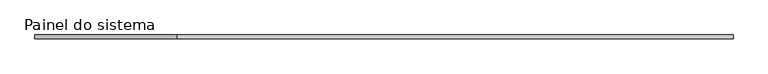
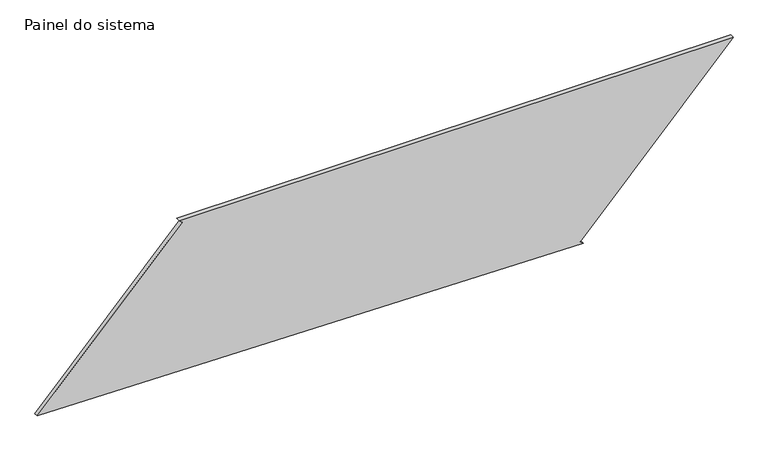
"""IFC4 building model written with IfcOpenShell, lengths in millimetres: plate geometry, Painel do sistema : Envidraçado."""

import ifcopenshell
import ifcopenshell.guid

model = None  # the IFC model being written
_history = None  # IfcOwnerHistory: only IFC2X3 demands one
_inside = {}  # id of a spatial element -> (the spatial element, [elements in it])
_under = {}  # id of a project, library or spatial element -> (it, [spatial elements below it])
_declared = {}  # id of a project -> (the project, [libraries it declares])
_typed = {}  # id of a type object -> (the type object, [elements of that type])
_made_of = {}  # id of a material, layer set ... -> (it, [elements and type objects made of it])


def new_model(schema):
    """Start an empty IFC model of exactly this schema.

    Asked for "IFC4X3", IfcOpenShell would pick the latest addendum, in which some entities
    have other attributes; the version numbers below select the first issue.
    IFC2X3 requires an IfcOwnerHistory on every rooted entity: one is made here for all.
    """
    global model, _history
    if schema == "IFC4X3":
        model = ifcopenshell.file(schema_version=(4, 3, 0, 0))
    else:
        model = ifcopenshell.file(schema=schema)
    _inside.clear()
    _under.clear()
    _declared.clear()
    _typed.clear()
    _made_of.clear()
    _history = None
    if model.schema == "IFC2X3":
        org = make("IfcOrganization", Name="unknown")
        user = make(
            "IfcPersonAndOrganization",
            ThePerson=make("IfcPerson", FamilyName="unknown"),
            TheOrganization=org,
        )
        app = make(
            "IfcApplication",
            ApplicationDeveloper=org,
            Version="unknown",
            ApplicationFullName="unknown",
            ApplicationIdentifier="unknown",
        )
        _history = make(
            "IfcOwnerHistory",
            OwningUser=user,
            OwningApplication=app,
            ChangeAction="ADDED",
            CreationDate=0,
        )
    return model


def make(cls, **values):
    """One entity of the class cls with the attributes given. An attribute that is None is left unset."""
    return model.create_entity(
        cls, **{name: value for name, value in values.items() if value is not None}
    )


def rooted(cls, **values):
    """An entity with a GlobalId (a new one), such as an element, a storey or a relation."""
    return make(cls, GlobalId=ifcopenshell.guid.new(), OwnerHistory=_history, **values)


def si_unit(unit_type, name, prefix=None):
    """IfcSIUnit, for example si_unit("LENGTHUNIT", "METRE", prefix="MILLI")."""
    return make("IfcSIUnit", UnitType=unit_type, Prefix=prefix, Name=name)


def assignment(units):
    """IfcUnitAssignment: the units of a project."""
    return None if units is None else make("IfcUnitAssignment", Units=units)


def point(xyz):
    """IfcCartesianPoint."""
    return None if xyz is None else make("IfcCartesianPoint", Coordinates=xyz)


def direction(xyz):
    """IfcDirection."""
    return None if xyz is None else make("IfcDirection", DirectionRatios=xyz)


def frame(location, z_axis=None, x_axis=None):
    """IfcAxis2Placement3D, a coordinate frame: its origin and axes. An axis left out is left unset."""
    return make(
        "IfcAxis2Placement3D",
        Location=point(location),
        Axis=direction(z_axis),
        RefDirection=direction(x_axis),
    )


def origin():
    """The frame at (0, 0, 0) with its axes left unset."""
    return frame((0.0, 0.0, 0.0))


def place(relative_to, where):
    """IfcLocalPlacement: puts the frame where relative to a parent placement (None: the world)."""
    return make(
        "IfcLocalPlacement", PlacementRelTo=relative_to, RelativePlacement=where
    )


def context(
    kind, dimensions, precision=None, world=None, true_north=None, identifier=None
):
    """IfcGeometricRepresentationContext, for example the 3D "Model" context."""
    return make(
        "IfcGeometricRepresentationContext",
        ContextIdentifier=identifier,
        ContextType=kind,
        CoordinateSpaceDimension=dimensions,
        Precision=precision,
        WorldCoordinateSystem=world,
        TrueNorth=true_north,
    )


def project(units=None, contexts=None):
    """IfcProject with its units and contexts."""
    return rooted(
        "IfcProject",
        Name="project",
        RepresentationContexts=contexts,
        UnitsInContext=assignment(units),
    )


def spatial(cls, under=None, at=None, **own):
    """A site, building, storey or space (cls), placed at a placement, below another one or the project."""
    s = rooted(cls, ObjectPlacement=at, **own)
    if under is not None:
        _under.setdefault(under.id(), (under, []))[1].append(s)
    return s


def polyline(points):
    """IfcPolyline through the points."""
    return make("IfcPolyline", Points=[point(p) for p in points])


def outline(outer, holes=None, kind="AREA"):
    """IfcArbitraryClosedProfileDef: a profile drawn as a closed curve; with holes, ...WithVoids."""
    if holes is None:
        return make("IfcArbitraryClosedProfileDef", ProfileType=kind, OuterCurve=outer)
    return make(
        "IfcArbitraryProfileDefWithVoids",
        ProfileType=kind,
        OuterCurve=outer,
        InnerCurves=holes,
    )


def extrude(swept, where, along, depth):
    """IfcExtrudedAreaSolid: the profile swept, set in the frame where, extruded along a direction by depth."""
    return make(
        "IfcExtrudedAreaSolid",
        SweptArea=swept,
        Position=where,
        ExtrudedDirection=direction(along),
        Depth=depth,
    )


def shape(context_of_items, identifier, shape_type, items):
    """IfcShapeRepresentation: the items that make up one representation, for example the "Body"."""
    return make(
        "IfcShapeRepresentation",
        ContextOfItems=context_of_items,
        RepresentationIdentifier=identifier,
        RepresentationType=shape_type,
        Items=items,
    )


def source(mapping_origin, context_of_items, identifier, shape_type, items):
    """IfcRepresentationMap: a shape defined once, which mapped items show again and again."""
    return make(
        "IfcRepresentationMap",
        MappingOrigin=mapping_origin,
        MappedRepresentation=shape(context_of_items, identifier, shape_type, items),
    )


def transform(
    local_origin,
    x_axis=None,
    y_axis=None,
    z_axis=None,
    scale=None,
    scale2=None,
    scale3=None,
    uniform=True,
):
    """IfcCartesianTransformationOperator3D, or its non-uniform kind. x_axis, y_axis, z_axis: its Axis1, 2, 3."""
    if uniform:
        return make(
            "IfcCartesianTransformationOperator3D",
            Axis1=direction(x_axis),
            Axis2=direction(y_axis),
            LocalOrigin=point(local_origin),
            Scale=scale,
            Axis3=direction(z_axis),
        )
    return make(
        "IfcCartesianTransformationOperator3DnonUniform",
        Axis1=direction(x_axis),
        Axis2=direction(y_axis),
        LocalOrigin=point(local_origin),
        Scale=scale,
        Axis3=direction(z_axis),
        Scale2=scale2,
        Scale3=scale3,
    )


def mapped(mapping_source, mapping_target):
    """IfcMappedItem: shows the shape of a source again, moved by a transform."""
    return make(
        "IfcMappedItem", MappingSource=mapping_source, MappingTarget=mapping_target
    )


def made_of(thing, what):
    """Note that an element or type object is made of a material, layer set ...; save() writes the relation."""
    if what is not None:
        _made_of.setdefault(what.id(), (what, []))[1].append(thing)
    return thing


def element(
    cls,
    number,
    at=None,
    inside=None,
    cuts=None,
    type_object=None,
    material=None,
    context=None,
    identifier="Body",
    shape_type=None,
    held_by="IfcProductDefinitionShape",
    body=None,
    shapes=None,
    **own,
):
    """One element of the class cls, such as IfcWall. Its Tag is "e" and its number.

    at: its placement. inside: the storey or other place that contains it. cuts: it is an
    opening in that element (IfcRelVoidsElement). A single representation is given by context,
    identifier, shape_type and body (its items); several are given by shapes. held_by: the class
    of the entity that holds the representations. save() writes the other relations.
    """
    e = rooted(cls, Tag="e%d" % number, ObjectPlacement=at, **own)
    if body is not None:
        shapes = [shape(context, identifier, shape_type, body)]
    if shapes is not None:
        e.Representation = make(held_by, Representations=shapes)
    if inside is not None:
        _inside.setdefault(inside.id(), (inside, []))[1].append(e)
    if cuts is not None:
        rooted(
            "IfcRelVoidsElement", RelatingBuildingElement=cuts, RelatedOpeningElement=e
        )
    if type_object is not None:
        _typed.setdefault(type_object.id(), (type_object, []))[1].append(e)
    return made_of(e, material)


def aggregate(whole, parts):
    """IfcRelAggregates: a whole, such as a stair, and the parts it consists of."""
    return rooted("IfcRelAggregates", RelatingObject=whole, RelatedObjects=parts)


def save(model, path):
    """Write the relations noted so far, then the file.

    IfcRelAggregates (storeys below a building ...), IfcRelContainedInSpatialStructure (elements
    in a storey), IfcRelDefinesByType, IfcRelAssociatesMaterial and IfcRelDeclares: one each for
    every whole, place, type object, material and project.
    """
    for whole, parts in _under.values():
        aggregate(whole, parts)
    for where, things in _inside.values():
        rooted(
            "IfcRelContainedInSpatialStructure",
            RelatedElements=things,
            RelatingStructure=where,
        )
    for kind, things in _typed.values():
        rooted("IfcRelDefinesByType", RelatedObjects=things, RelatingType=kind)
    for what, things in _made_of.values():
        rooted("IfcRelAssociatesMaterial", RelatedObjects=things, RelatingMaterial=what)
    for by, libraries in _declared.values():
        rooted("IfcRelDeclares", RelatingContext=by, RelatedDefinitions=libraries)
    model.write(path)


def painel_do_sistema_a36432ed(model_context):
    return source(origin(), model_context, "Body", "SweptSolid", [
        extrude(outline(polyline([(0.0, 1249.6137431), (17.1196584, 1231.3951455), (1043.5319173, 2195.8945903), (1043.5319173, -1300.023427), (1026.4122589, -1281.8048294), (53.6455649, -2195.8945903), (0.0, 1249.6137431)])), frame((0.0, 24.5, 0.0), z_axis=(0.0, 1.0, 0.0), x_axis=(0.0, 0.0, 1.0)), (0.0, 0.0, 1.0), 25.0),
    ])


if __name__ == "__main__":
    model = new_model("IFC4")
    model_context = context("Model", 3, world=origin())
    ifc_project = project(units=[si_unit("LENGTHUNIT", "METRE", prefix="MILLI")], contexts=[model_context])
    site = spatial("IfcSite", under=ifc_project)
    building = spatial("IfcBuilding", under=site)
    placement = place(None, origin())
    painel_do_sistema_shape = painel_do_sistema_a36432ed(model_context)
    element("IfcPlate", 1, ObjectType="Painel do sistema : Envidraçado", at=placement, inside=building, context=model_context, shape_type="MappedRepresentation", body=[
        mapped(painel_do_sistema_shape, transform((0.0, 0.0, 0.0), x_axis=(1.0, 0.0, 0.0), y_axis=(0.0, 1.0, 0.0), z_axis=(0.0, 0.0, 1.0))),
    ])
    save(model, "model.ifc")

# Revit data of these elements
# Type "Painel do sistema : Envidraçado"
#   Construction Type Id = "GSP4R"
#   Analytic Construction = "Vidraça única Pilkington 1/8 pol"
#   Visual Light Transmittance = 0.9
#   Solar Heat Gain Coefficient = 0.86
#   Heat Transfer Coefficient (U) = 6.7069 W/(m²·K)
# Element 1 (IfcPlate, "Painel do sistema : Envidraçado")
#   Materials on its faces: "Vidro"
# Materials
#   "Vidro": class "Vidro", colour RGB 0 128 192, transparency 0.9, Description = "Vidro de sílica", Cost = 0
